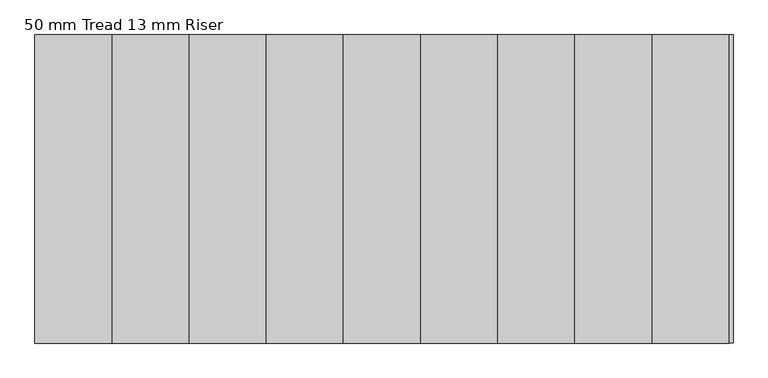
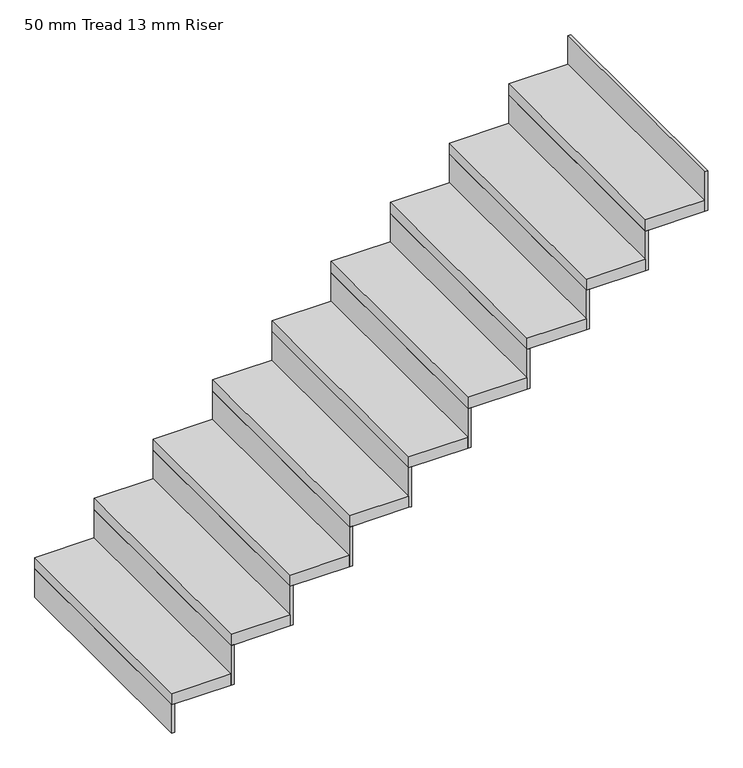
"""IFC4 building model written with IfcOpenShell, lengths in millimetres: stair flight geometry, 50 mm Tread 13 mm Riser."""

from ifc_helpers import new_model, si_unit, frame, origin, origin_with_axes, place, context, project, spatial, polyline, outline, extrude, source, transform, mapped, element, save


def stair_flight_50_mm_tread_13_mm_riser_45536860(model_context):
    return source(origin(), model_context, "Body", "SweptSolid", [
        extrude(outline(polyline([(28456.6667192, -4197.3716232), (28444.1667192, -4197.3716232), (28444.1667192, -3197.3716232), (28456.6667192, -3197.3716232), (28456.6667192, -4197.3716232)])), origin_with_axes(), (0.0, 0.0, 1.0), 126.4705882),
        extrude(outline(polyline([(28694.1667192, -3197.3716232), (28694.1667192, -4197.3716232), (28444.1667192, -4197.3716232), (28444.1667192, -3197.3716232), (28694.1667192, -3197.3716232)])), frame((0.0, 0.0, 126.4705882), z_axis=(0.0, 0.0, 1.0), x_axis=(1.0, 0.0, 0.0)), (0.0, 0.0, 1.0), 50.0),
        extrude(outline(polyline([(28706.6667192, -4197.3716232), (28694.1667192, -4197.3716232), (28694.1667192, -3197.3716232), (28706.6667192, -3197.3716232), (28706.6667192, -4197.3716232)])), frame((0.0, 0.0, 126.4705882), z_axis=(0.0, 0.0, 1.0), x_axis=(1.0, 0.0, 0.0)), (0.0, 0.0, 1.0), 176.4705882),
        extrude(outline(polyline([(28944.1667192, -3197.3716232), (28944.1667192, -4197.3716232), (28694.1667192, -4197.3716232), (28694.1667192, -3197.3716232), (28944.1667192, -3197.3716232)])), frame((0.0, 0.0, 302.9411765), z_axis=(0.0, 0.0, 1.0), x_axis=(1.0, 0.0, 0.0)), (0.0, 0.0, 1.0), 50.0),
        extrude(outline(polyline([(28956.6667192, -4197.3716232), (28944.1667192, -4197.3716232), (28944.1667192, -3197.3716232), (28956.6667192, -3197.3716232), (28956.6667192, -4197.3716232)])), frame((0.0, 0.0, 302.9411765), z_axis=(0.0, 0.0, 1.0), x_axis=(1.0, 0.0, 0.0)), (0.0, 0.0, 1.0), 176.4705882),
        extrude(outline(polyline([(29194.1667192, -3197.3716232), (29194.1667192, -4197.3716232), (28944.1667192, -4197.3716232), (28944.1667192, -3197.3716232), (29194.1667192, -3197.3716232)])), frame((0.0, 0.0, 479.4117647), z_axis=(0.0, 0.0, 1.0), x_axis=(1.0, 0.0, 0.0)), (0.0, 0.0, 1.0), 50.0),
        extrude(outline(polyline([(29206.6667192, -4197.3716232), (29194.1667192, -4197.3716232), (29194.1667192, -3197.3716232), (29206.6667192, -3197.3716232), (29206.6667192, -4197.3716232)])), frame((0.0, 0.0, 479.4117647), z_axis=(0.0, 0.0, 1.0), x_axis=(1.0, 0.0, 0.0)), (0.0, 0.0, 1.0), 176.4705882),
        extrude(outline(polyline([(29444.1667192, -3197.3716232), (29444.1667192, -4197.3716232), (29194.1667192, -4197.3716232), (29194.1667192, -3197.3716232), (29444.1667192, -3197.3716232)])), frame((0.0, 0.0, 655.8823529), z_axis=(0.0, 0.0, 1.0), x_axis=(1.0, 0.0, 0.0)), (0.0, 0.0, 1.0), 50.0),
        extrude(outline(polyline([(29456.6667192, -4197.3716232), (29444.1667192, -4197.3716232), (29444.1667192, -3197.3716232), (29456.6667192, -3197.3716232), (29456.6667192, -4197.3716232)])), frame((0.0, 0.0, 655.8823529), z_axis=(0.0, 0.0, 1.0), x_axis=(1.0, 0.0, 0.0)), (0.0, 0.0, 1.0), 176.4705882),
        extrude(outline(polyline([(29694.1667192, -3197.3716232), (29694.1667192, -4197.3716232), (29444.1667192, -4197.3716232), (29444.1667192, -3197.3716232), (29694.1667192, -3197.3716232)])), frame((0.0, 0.0, 832.3529412), z_axis=(0.0, 0.0, 1.0), x_axis=(1.0, 0.0, 0.0)), (0.0, 0.0, 1.0), 50.0),
        extrude(outline(polyline([(29706.6667192, -4197.3716232), (29694.1667192, -4197.3716232), (29694.1667192, -3197.3716232), (29706.6667192, -3197.3716232), (29706.6667192, -4197.3716232)])), frame((0.0, 0.0, 832.3529412), z_axis=(0.0, 0.0, 1.0), x_axis=(1.0, 0.0, 0.0)), (0.0, 0.0, 1.0), 176.4705882),
        extrude(outline(polyline([(29944.1667192, -3197.3716232), (29944.1667192, -4197.3716232), (29694.1667192, -4197.3716232), (29694.1667192, -3197.3716232), (29944.1667192, -3197.3716232)])), frame((0.0, 0.0, 1008.8235294), z_axis=(0.0, 0.0, 1.0), x_axis=(1.0, 0.0, 0.0)), (0.0, 0.0, 1.0), 50.0),
        extrude(outline(polyline([(29956.6667192, -4197.3716232), (29944.1667192, -4197.3716232), (29944.1667192, -3197.3716232), (29956.6667192, -3197.3716232), (29956.6667192, -4197.3716232)])), frame((0.0, 0.0, 1008.8235294), z_axis=(0.0, 0.0, 1.0), x_axis=(1.0, 0.0, 0.0)), (0.0, 0.0, 1.0), 176.4705882),
        extrude(outline(polyline([(30194.1667192, -3197.3716232), (30194.1667192, -4197.3716232), (29944.1667192, -4197.3716232), (29944.1667192, -3197.3716232), (30194.1667192, -3197.3716232)])), frame((0.0, 0.0, 1185.2941176), z_axis=(0.0, 0.0, 1.0), x_axis=(1.0, 0.0, 0.0)), (0.0, 0.0, 1.0), 50.0),
        extrude(outline(polyline([(30206.6667192, -4197.3716232), (30194.1667192, -4197.3716232), (30194.1667192, -3197.3716232), (30206.6667192, -3197.3716232), (30206.6667192, -4197.3716232)])), frame((0.0, 0.0, 1185.2941176), z_axis=(0.0, 0.0, 1.0), x_axis=(1.0, 0.0, 0.0)), (0.0, 0.0, 1.0), 176.4705882),
        extrude(outline(polyline([(30444.1667192, -3197.3716232), (30444.1667192, -4197.3716232), (30194.1667192, -4197.3716232), (30194.1667192, -3197.3716232), (30444.1667192, -3197.3716232)])), frame((0.0, 0.0, 1361.7647059), z_axis=(0.0, 0.0, 1.0), x_axis=(1.0, 0.0, 0.0)), (0.0, 0.0, 1.0), 50.0),
        extrude(outline(polyline([(30456.6667192, -4197.3716232), (30444.1667192, -4197.3716232), (30444.1667192, -3197.3716232), (30456.6667192, -3197.3716232), (30456.6667192, -4197.3716232)])), frame((0.0, 0.0, 1361.7647059), z_axis=(0.0, 0.0, 1.0), x_axis=(1.0, 0.0, 0.0)), (0.0, 0.0, 1.0), 176.4705882),
        extrude(outline(polyline([(30706.6667192, -4197.3716232), (30694.1667192, -4197.3716232), (30694.1667192, -3197.3716232), (30706.6667192, -3197.3716232), (30706.6667192, -4197.3716232)])), frame((0.0, 0.0, 1538.2352941), z_axis=(0.0, 0.0, 1.0), x_axis=(1.0, 0.0, 0.0)), (0.0, 0.0, 1.0), 176.4705882),
        extrude(outline(polyline([(30694.1667192, -3197.3716232), (30694.1667192, -4197.3716232), (30444.1667192, -4197.3716232), (30444.1667192, -3197.3716232), (30694.1667192, -3197.3716232)])), frame((0.0, 0.0, 1538.2352941), z_axis=(0.0, 0.0, 1.0), x_axis=(1.0, 0.0, 0.0)), (0.0, 0.0, 1.0), 50.0),
    ])


if __name__ == "__main__":
    model = new_model("IFC4")
    model_context = context("Model", 3, world=origin())
    ifc_project = project(units=[si_unit("LENGTHUNIT", "METRE", prefix="MILLI")], contexts=[model_context])
    site = spatial("IfcSite", under=ifc_project)
    building = spatial("IfcBuilding", under=site)
    placement = place(None, origin())
    stair_flight_50_mm_tread_13_mm_riser_shape = stair_flight_50_mm_tread_13_mm_riser_45536860(model_context)
    element("IfcStairFlight", 1, ObjectType="50 mm Tread 13 mm Riser", at=placement, inside=building, context=model_context, shape_type="MappedRepresentation", body=[
        mapped(stair_flight_50_mm_tread_13_mm_riser_shape, transform((0.0, 0.0, 0.0), x_axis=(1.0, 0.0, 0.0), y_axis=(0.0, 1.0, 0.0), z_axis=(0.0, 0.0, 1.0))),
    ])
    save(model, "model.ifc")
